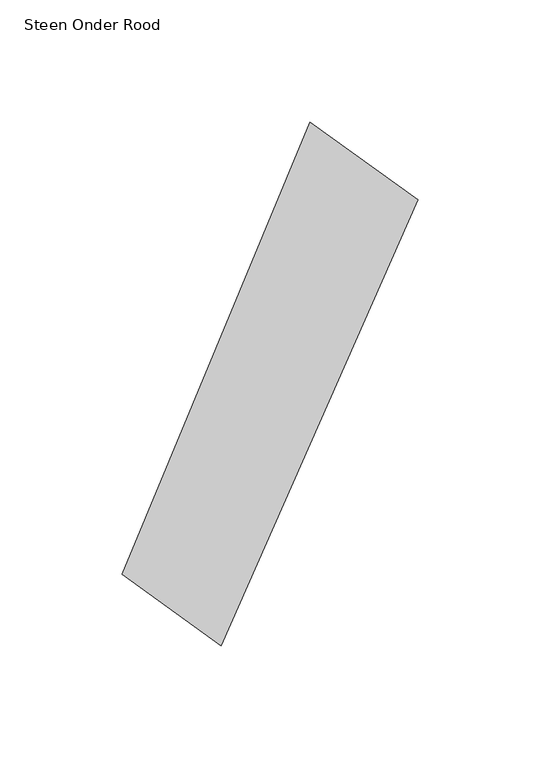
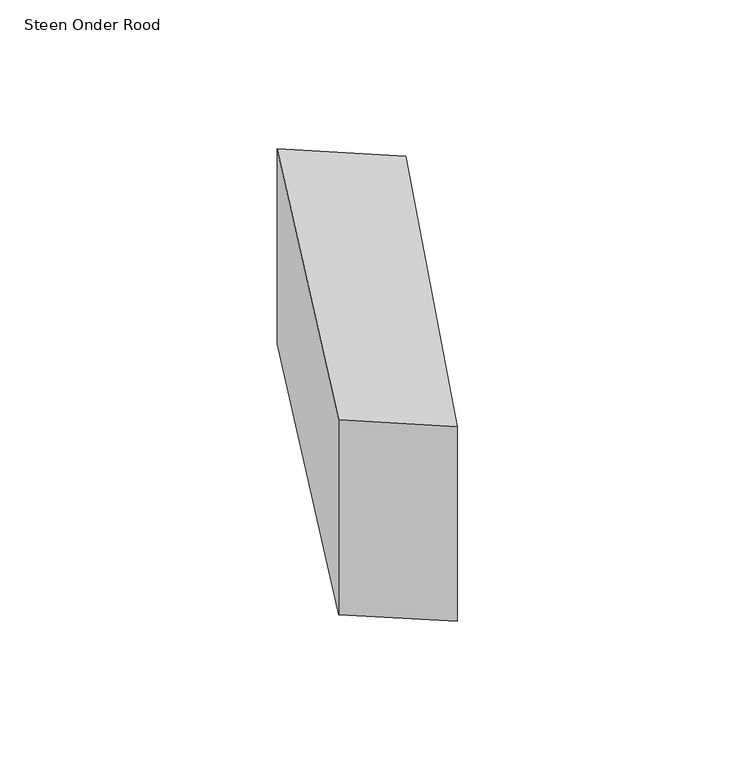
"""IFC4 building model written with IfcOpenShell, lengths in millimetres: proxy geometry, 00_GMA_steen_versie_4 : Steen Onder Rood."""

from ifc_helpers import new_model, si_unit, origin, origin_with_axes, place, context, project, spatial, polyline, outline, extrude, source, transform, mapped, element, save


def steen_onder_rood_43e1f348(model_context):
    return source(origin(), model_context, "Body", "SweptSolid", [
        extrude(outline(polyline([(140.7370054, 160.4486557), (60.234068, -21.9892992), (19.6455199, 7.209498), (96.6358143, 192.1982895), (140.7370054, 160.4486557)])), origin_with_axes(), (0.0, 0.0, 1.0), 100.0),
    ])


if __name__ == "__main__":
    model = new_model("IFC4")
    model_context = context("Model", 3, world=origin())
    ifc_project = project(units=[si_unit("LENGTHUNIT", "METRE", prefix="MILLI")], contexts=[model_context])
    site = spatial("IfcSite", under=ifc_project)
    building = spatial("IfcBuilding", under=site)
    placement = place(None, origin())
    steen_onder_rood_shape = steen_onder_rood_43e1f348(model_context)
    element("IfcBuildingElementProxy", 1, Name="00_GMA_steen_versie_4 : Steen Onder Rood", ObjectType="00_GMA_steen_versie_4 : Steen Onder Rood", at=placement, inside=building, context=model_context, shape_type="MappedRepresentation", body=[
        mapped(steen_onder_rood_shape, transform((0.0, 0.0, 0.0), x_axis=(1.0, 0.0, 0.0), y_axis=(0.0, 1.0, 0.0), z_axis=(0.0, 0.0, 1.0))),
    ])
    save(model, "model.ifc")

# Revit data of these elements
# Type "00_GMA_steen_versie_4 : Steen Onder Rood"
#   StootVoegHalfBoven [instance default] = 5 mm
#   StootVoegHalf [instance default] = 5 mm
#   StootVoegBreedteOnder = 10 mm
#   StootVoegBreedteBoven = 10 mm
#   Steendikte = 100 mm
#   LintVoegOnderHalf = 0 mm
#   LintVoegOnder = 0 mm
#   LintVoegBovenHalf = 5 mm
#   LintVoegBoven = 10 mm
#   materiaal = 21_steen_rood
#   MateriaalVoeg = none
#   Default Elevation = 0
# Element 1 (IfcBuildingElementProxy, "00_GMA_steen_versie_4 : Steen Onder Rood")
#   Materials on its faces: "21_steen_rood"
# Materials
#   "21_steen_rood": class "Unassigned", colour RGB 213 111 43, transparency 0, Cost = 0
